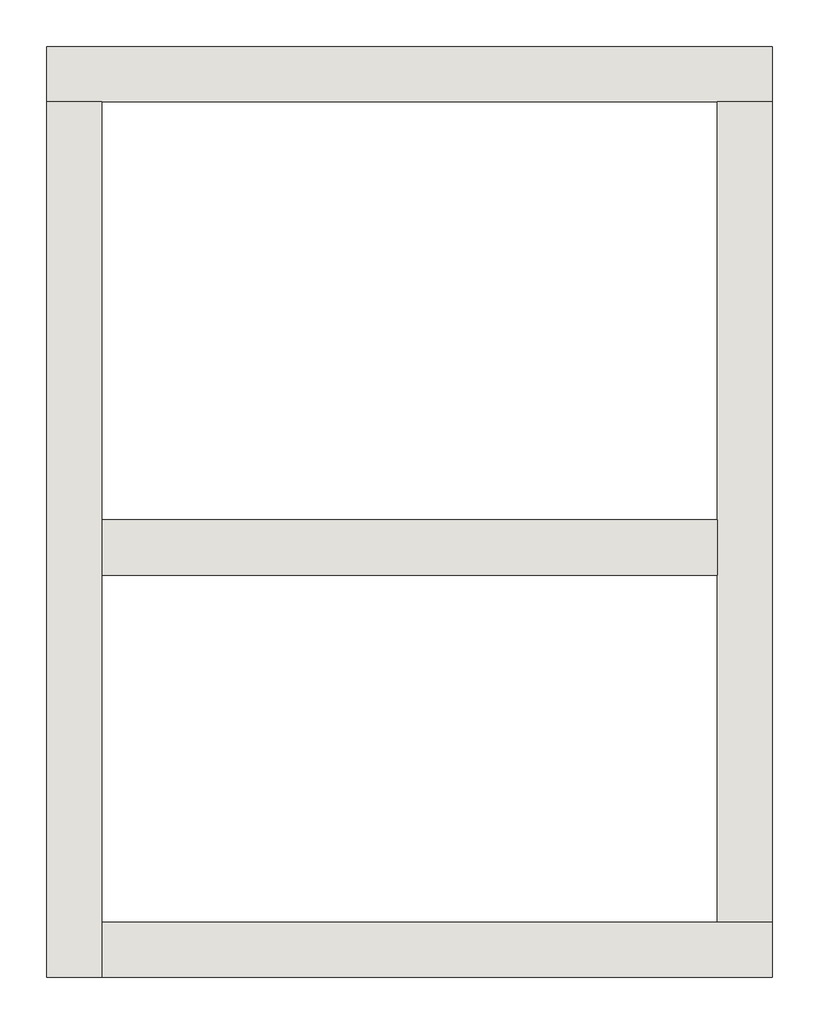
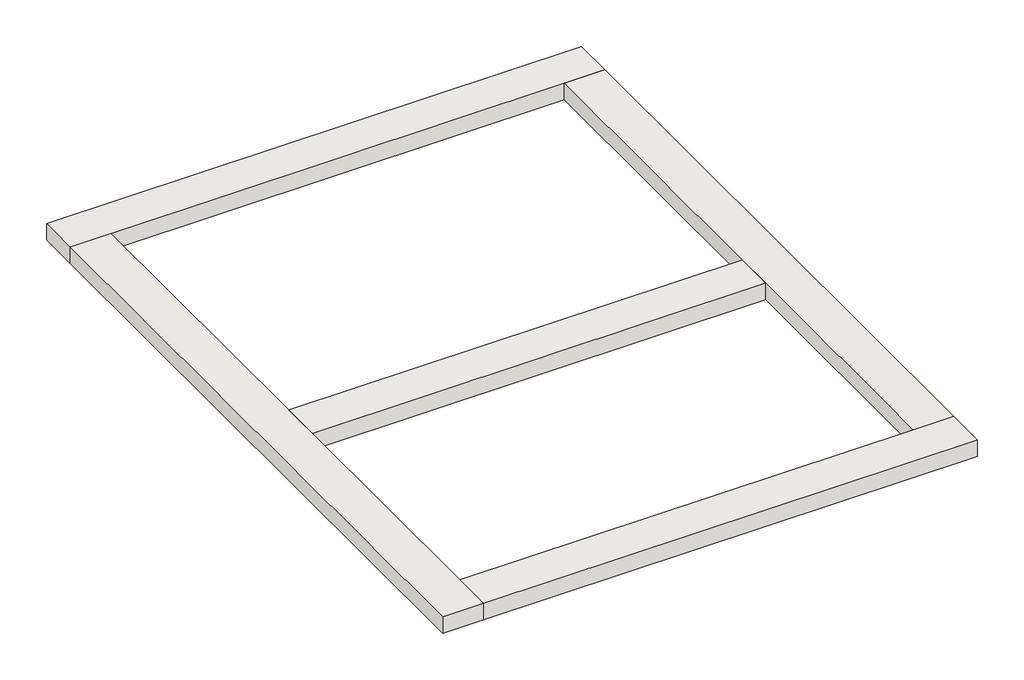
# One storey: 5 walls.
"""IFC4 building model written with IfcOpenShell, lengths in millimetres."""

from ifc_helpers import new_model, si_unit, frame, origin, place, context, project, spatial, polyline, outline, extrude, faceted_brep, element, save

model = new_model("IFC4")

# Units and contexts
model_context = context("Model", 3, world=origin())
ifc_project = project(units=[si_unit("LENGTHUNIT", "METRE", prefix="MILLI")], contexts=[model_context])

# Site, building, storey
site = spatial("IfcSite", under=ifc_project)
building = spatial("IfcBuilding", under=site)
storey = spatial("IfcBuildingStorey", under=building, Name="ЛФ", Elevation=-300.0)

# Walls
placement = place(None, origin())
element("IfcWall", 1, ObjectType="Ленточный Фундамент - Бетон 700х300", at=placement, inside=storey, context=model_context, shape_type="Brep", body=[
    faceted_brep([(-10030.6631644, -1872.3774925, -300.0), (-19230.6631644, -1872.3774925, -300.0), (-19230.6631644, -1872.3774925, 0.0), (-10030.6631644, -1872.3774925, 0.0), (-10030.6631644, -2572.3774925, -300.0), (-10030.6631644, -2572.3774925, 0.0), (-10730.6631644, -2572.3774925, 0.0), (-18530.6631644, -2572.3774925, 0.0), (-19230.6631644, -2572.3774925, 0.0), (-19230.6631644, -2572.3774925, -300.0), (-18530.6631644, -2572.3774925, -300.0), (-10730.6631644, -2572.3774925, -300.0)], [[[0, 1, 2, 3]], [[4, 5, 6, 7, 8, 9, 10, 11]], [[1, 0, 4, 11, 10, 9]], [[3, 2, 8, 7, 6, 5]], [[2, 1, 9, 8]], [[0, 3, 5, 4]]]),
])
element("IfcWall", 2, ObjectType="Ленточный Фундамент - Бетон 700х300", at=placement, inside=storey, context=model_context, shape_type="Brep", body=[
    faceted_brep([(-19230.6631644, -2572.3774925, -300.0), (-19230.6631644, -13672.3774925, -300.0), (-19230.6631644, -13672.3774925, 0.0), (-19230.6631644, -2572.3774925, 0.0), (-18530.6631644, -2572.3774925, -300.0), (-18530.6631644, -2572.3774925, 0.0), (-18530.6631644, -7872.3774925, 0.0), (-18530.6631644, -8572.3774925, 0.0), (-18530.6631644, -12972.3774925, 0.0), (-18530.6631644, -13672.3774925, 0.0), (-18530.6631644, -13672.3774925, -300.0), (-18530.6631644, -12972.3774925, -300.0), (-18530.6631644, -8572.3774925, -300.0), (-18530.6631644, -7872.3774925, -300.0)], [[[0, 1, 2, 3]], [[4, 5, 6, 7, 8, 9, 10, 11, 12, 13]], [[1, 0, 4, 13, 12, 11, 10]], [[3, 2, 9, 8, 7, 6, 5]], [[0, 3, 5, 4]], [[2, 1, 10, 9]]]),
])
element("IfcWall", 3, ObjectType="Ленточный Фундамент - Бетон 700х300", at=placement, inside=storey, context=model_context, shape_type="SweptSolid", body=[
    extrude(outline(polyline([(-10730.6631644, -8572.3774925), (-18530.6631644, -8572.3774925), (-18530.6631644, -7872.3774925), (-10730.6631644, -7872.3774925), (-10730.6631644, -8572.3774925)])), frame((0.0, 0.0, -300.0), z_axis=(0.0, 0.0, 1.0), x_axis=(1.0, 0.0, 0.0)), (0.0, 0.0, 1.0), 300.0),
])
element("IfcWall", 4, ObjectType="Ленточный Фундамент - Бетон 700х300", at=placement, inside=storey, context=model_context, shape_type="Brep", body=[
    faceted_brep([(-10030.6631644, -12972.3774925, -300.0), (-10030.6631644, -2572.3774925, -300.0), (-10030.6631644, -2572.3774925, 0.0), (-10030.6631644, -12972.3774925, 0.0), (-10730.6631644, -12972.3774925, -300.0), (-10730.6631644, -12972.3774925, 0.0), (-10730.6631644, -8572.3774925, 0.0), (-10730.6631644, -7872.3774925, 0.0), (-10730.6631644, -2572.3774925, 0.0), (-10730.6631644, -2572.3774925, -300.0), (-10730.6631644, -7872.3774925, -300.0), (-10730.6631644, -8572.3774925, -300.0)], [[[0, 1, 2, 3]], [[4, 5, 6, 7, 8, 9, 10, 11]], [[1, 0, 4, 11, 10, 9]], [[3, 2, 8, 7, 6, 5]], [[2, 1, 9, 8]], [[0, 3, 5, 4]]]),
])
element("IfcWall", 5, ObjectType="Ленточный Фундамент - Бетон 700х300", at=placement, inside=storey, context=model_context, shape_type="Brep", body=[
    faceted_brep([(-18530.6631644, -13672.3774925, -300.0), (-10030.6631644, -13672.3774925, -300.0), (-10030.6631644, -13672.3774925, 0.0), (-18530.6631644, -13672.3774925, 0.0), (-18530.6631644, -12972.3774925, -300.0), (-18530.6631644, -12972.3774925, 0.0), (-10730.6631644, -12972.3774925, 0.0), (-10030.6631644, -12972.3774925, 0.0), (-10030.6631644, -12972.3774925, -300.0), (-10730.6631644, -12972.3774925, -300.0)], [[[0, 1, 2, 3]], [[4, 5, 6, 7, 8, 9]], [[1, 0, 4, 9, 8]], [[3, 2, 7, 6, 5]], [[0, 3, 5, 4]], [[2, 1, 8, 7]]]),
])

save(model, "model.ifc")

# Revit data of these elements
# Project information
#   Дата утверждения проекта = "Дата выпуска"
#   Статус проекта = "Статус проекта"
#   Заказчик = "Владелец"
#   Адрес проекта = "Укажите адрес"
#   Наименование проекта = "Наименование проекта"
#   Номер проекта = "0001"
# Grids (mm)
#   "Г": line (-4340.98, -20022.377) -> (-25012.719, -20022.377)
#   "2": line (-17080.663, -10863.582) -> (-17080.663, -22509.536)
#   "3": line (-12080.663, -10863.582) -> (-12080.663, -22509.536)
#   "К2": line (-4521.619, -15522.377) -> (-25012.719, -15522.377)
#   "А": line (-25012.719, -13322.377) -> (-1373.536, -13322.377)
#   "Б": line (-25012.719, -8222.377) -> (-1373.536, -8222.377)
#   "В": line (-25012.719, -2222.377) -> (-1373.536, -2222.377)
#   "1": line (-18880.663, -22509.536) -> (-18880.663, 58.421)
#   "4": line (-10380.663, -22509.536) -> (-10380.663, 58.421)
#   "К1": line (-8180.663, -17421.308) -> (-8180.663, -10643.103)
# Type "Ленточный Фундамент - Бетон 700х300"
#   Layers, outside or top first: 700 mm "Бетон, монолитный" (function 1)
# Elements 1, 2, 3, 4, 5 (IfcWall, "Ленточный Фундамент - Бетон 700х300")
#   Top Offset = 0 mm
#   Base Offset = 0 mm
#   wall height = 300 mm
#   Phase Created = Новая конструкция
#   Base Constraint = ЛФ
#   Top Constraint = Уровень 1
#   Materials on its faces: "Бетон, монолитный"
# Materials
#   "Бетон, монолитный": class "Бетон", colour RGB 192 192 192, transparency 0, Description = "физический материал", Cost = 0
